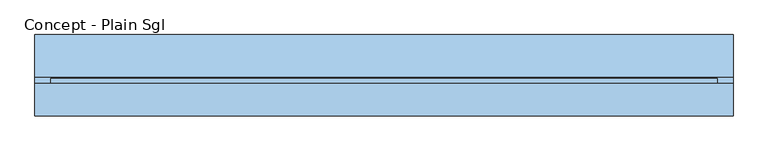
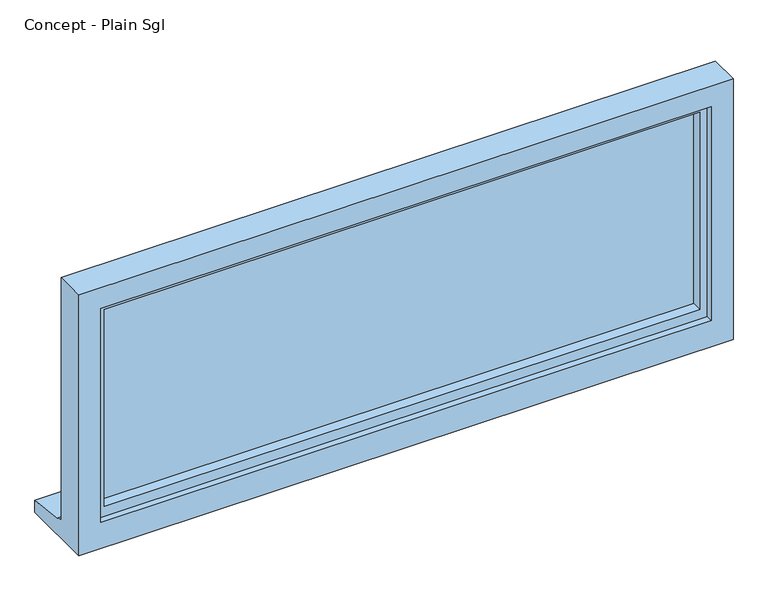
"""IFC4 building model written with IfcOpenShell, lengths in millimetres: window geometry, Concept - Plain Sgl : Dormer Window 1777w x 650mmh No Opening Sashes."""

from ifc_helpers import new_model, si_unit, frame, origin, place, context, project, spatial, polyline, outline, extrude, faceted_brep, source, transform, mapped, element, save


def concept_plain_sgl_b2c60465(model_context):
    return source(origin(), model_context, "Body", "SolidModel", [
        faceted_brep([(-889.0, -10.7934322, 1360.0), (889.0, -10.7934322, 1360.0), (889.0, -10.7934322, 2110.0), (-889.0, -10.7934322, 2110.0), (-829.0, -10.7934322, 2050.0), (829.0, -10.7934322, 2050.0), (829.0, -10.7934322, 1435.0), (-829.0, -10.7934322, 1435.0), (-889.0, 72.2065678, 2110.0), (-889.0, 72.2065678, 1411.0), (-889.0, 87.2065678, 1409.68767), (-889.0, 87.2065678, 1404.7449676), (-889.0, 195.9565678, 1393.8088847), (-889.0, 195.9565678, 1360.0), (889.0, 72.2065678, 2110.0), (889.0, 72.2065678, 1411.0), (-849.0, 72.2065678, 2070.0), (-849.0, 72.2065678, 1423.0), (849.0, 72.2065678, 1423.0), (849.0, 72.2065678, 2070.0), (-849.0, 7.2065678, 2070.0), (-849.0, 7.2065678, 1423.0), (849.0, 7.2065678, 2070.0), (849.0, 7.2065678, 1423.0), (-829.0, 7.2065678, 2050.0), (-829.0, 7.2065678, 1435.0), (829.0, 7.2065678, 1435.0), (829.0, 7.2065678, 2050.0), (889.0, 195.9565678, 1360.0), (889.0, 195.9565678, 1393.8088847), (889.0, 87.2065678, 1404.7449676), (889.0, 87.2065678, 1409.68767)], [[[0, 1, 2, 3], [4, 5, 6, 7]], [[0, 3, 8, 9, 10, 11, 12, 13]], [[9, 8, 14, 15], [16, 17, 18, 19]], [[17, 16, 20, 21]], [[20, 22, 23, 21], [24, 25, 26, 27]], [[24, 4, 7, 25]], [[3, 2, 14, 8]], [[16, 19, 22, 20]], [[5, 4, 24, 27]], [[15, 14, 2, 1, 28, 29, 30, 31]], [[19, 18, 23, 22]], [[5, 27, 26, 6]], [[28, 1, 0, 13]], [[29, 28, 13, 12]], [[30, 29, 12, 11]], [[31, 30, 11, 10]], [[15, 31, 10, 9]], [[21, 23, 18, 17]], [[7, 6, 26, 25]]]),
        extrude(outline(polyline([(819.0, 36.2065678), (-819.0, 36.2065678), (-819.0, 60.2065678), (819.0, 60.2065678), (819.0, 36.2065678)])), frame((0.0, 0.0, 1453.0), z_axis=(0.0, 0.0, 1.0), x_axis=(1.0, 0.0, 0.0)), (0.0, 0.0, 1.0), 587.0),
        faceted_brep([(-849.0, 7.2065678, 2070.0), (-849.0, 83.7535732, 2070.0), (-849.0, 83.7535732, 1423.0), (-849.0, 7.2065678, 1423.0), (-809.0, 36.2065678, 2030.0), (-809.0, 7.2065678, 2030.0), (-809.0, 7.2065678, 1463.0), (-809.0, 36.2065678, 1463.0), (-819.0, 60.2065678, 2040.0), (-819.0, 36.2065678, 2040.0), (-819.0, 36.2065678, 1453.0), (-819.0, 60.2065678, 1453.0), (-809.0, 83.7535732, 2030.0), (-809.0, 60.2065678, 2030.0), (-809.0, 60.2065678, 1463.0), (-809.0, 83.7535732, 1463.0), (849.0, 83.7535732, 1423.0), (849.0, 7.2065678, 1423.0), (809.0, 7.2065678, 1463.0), (809.0, 36.2065678, 1463.0), (819.0, 36.2065678, 1453.0), (819.0, 60.2065678, 1453.0), (809.0, 60.2065678, 1463.0), (809.0, 83.7535732, 1463.0), (849.0, 83.7535732, 2070.0), (849.0, 7.2065678, 2070.0), (809.0, 7.2065678, 2030.0), (809.0, 36.2065678, 2030.0), (819.0, 36.2065678, 2040.0), (819.0, 60.2065678, 2040.0), (809.0, 60.2065678, 2030.0), (809.0, 83.7535732, 2030.0)], [[[0, 1, 2, 3]], [[4, 5, 6, 7]], [[8, 9, 10, 11]], [[12, 13, 14, 15]], [[3, 2, 16, 17]], [[7, 6, 18, 19]], [[11, 10, 20, 21]], [[15, 14, 22, 23]], [[17, 16, 24, 25]], [[19, 18, 26, 27]], [[21, 20, 28, 29]], [[23, 22, 30, 31]], [[1, 24, 16, 2], [15, 23, 31, 12]], [[25, 24, 1, 0]], [[3, 17, 25, 0], [5, 26, 18, 6]], [[27, 26, 5, 4]], [[9, 28, 20, 10], [7, 19, 27, 4]], [[29, 28, 9, 8]], [[11, 21, 29, 8], [13, 30, 22, 14]], [[31, 30, 13, 12]]]),
    ])


if __name__ == "__main__":
    model = new_model("IFC4")
    model_context = context("Model", 3, world=origin())
    ifc_project = project(units=[si_unit("LENGTHUNIT", "METRE", prefix="MILLI")], contexts=[model_context])
    site = spatial("IfcSite", under=ifc_project)
    building = spatial("IfcBuilding", under=site)
    placement = place(None, origin())
    concept_plain_sgl_shape = concept_plain_sgl_b2c60465(model_context)
    element("IfcWindow", 1, ObjectType="Concept - Plain Sgl : Dormer Window 1777w x 650mmh No Opening Sashes", at=placement, inside=building, context=model_context, shape_type="MappedRepresentation", body=[
        mapped(concept_plain_sgl_shape, transform((0.0, 0.0, 0.0), x_axis=(1.0, 0.0, 0.0), y_axis=(0.0, 1.0, 0.0), z_axis=(0.0, 0.0, 1.0))),
    ])
    save(model, "model.ifc")

# Revit data of these elements
# Type "Concept - Plain Sgl : Dormer Window 1777w x 650mmh No Opening Sashes"
#   Description = "Dormer Window - No Opening Sash Vents"
#   Type Mark = "59"
#   Operation = "SinglePanel"
#   Manufacturer = "Revit"
#   Keynote = "L10"
#   Visual Light Transmittance = 0.9
#   Solar Heat Gain Coefficient = 0.86
#   Rough Width = 1778 mm
#   Rough Height = 750 mm
#   Height = 750 mm
#   Width = 1778 mm
#   Heat Transfer Coefficient (U) = 5.5617 W/(m²·K)
#   FrameOffset - External = 0 mm
#   Default Head Height = 2110 mm
#   Material Trim = Window Frame
#   Material Glass = Glass
#   Material Frame = Window Frame
#   Construction Type Id = ""
#   Wall Closure = (empty or 0)
#   Analytic Construction = (empty or 0)
# Element 1 (IfcWindow, "Concept - Plain Sgl : Dormer Window 1777w x 650mmh No Opening Sashes")
#   Materials on its faces: "Window Frame", "Glass"
# Materials
#   "Window Frame": class "Miscellaneous", colour RGB 249 249 249, transparency 0, Keynote = "L10"
#   "Glass": class "Glass", colour RGB 0 128 192, transparency 0.9, Description = "Soda Lime Glass", Cost = 0
